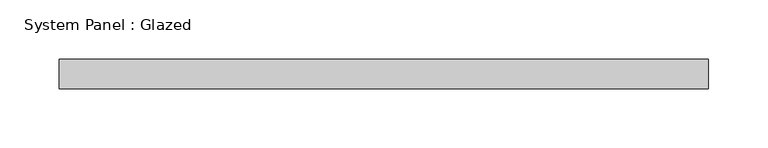
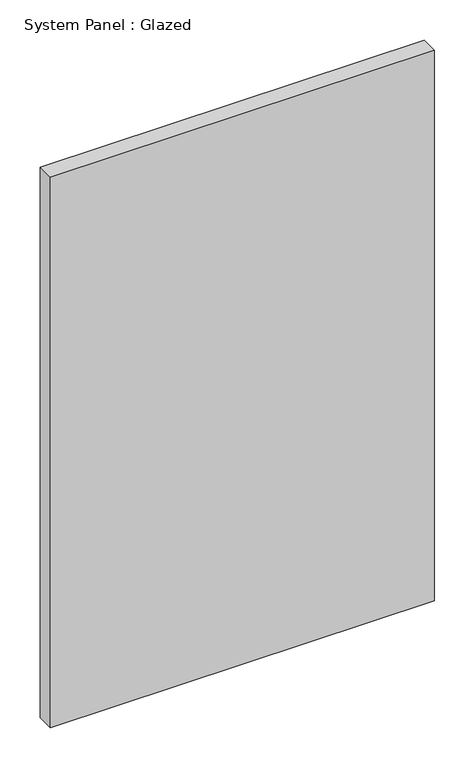
"""IFC4 building model written with IfcOpenShell, lengths in millimetres: plate geometry, System Panel : Glazed."""

from ifc_helpers import new_model, si_unit, origin, origin_with_axes, place, context, project, spatial, polyline, outline, extrude, source, transform, mapped, element, save


def system_panel_glazed_fb5ef4b2(model_context):
    return source(origin(), model_context, "Body", "SweptSolid", [
        extrude(outline(polyline([(275.0, 24.5), (-275.0, 24.5), (-275.0, 49.5), (275.0, 49.5), (275.0, 24.5)])), origin_with_axes(), (0.0, 0.0, 1.0), 833.3333333),
    ])


if __name__ == "__main__":
    model = new_model("IFC4")
    model_context = context("Model", 3, world=origin())
    ifc_project = project(units=[si_unit("LENGTHUNIT", "METRE", prefix="MILLI")], contexts=[model_context])
    site = spatial("IfcSite", under=ifc_project)
    building = spatial("IfcBuilding", under=site)
    placement = place(None, origin())
    system_panel_glazed_shape = system_panel_glazed_fb5ef4b2(model_context)
    element("IfcPlate", 1, ObjectType="System Panel : Glazed", at=placement, inside=building, context=model_context, shape_type="MappedRepresentation", body=[
        mapped(system_panel_glazed_shape, transform((0.0, 0.0, 0.0), x_axis=(1.0, 0.0, 0.0), y_axis=(0.0, 1.0, 0.0), z_axis=(0.0, 0.0, 1.0))),
    ])
    save(model, "model.ifc")

# Revit data of these elements
# Element 1 (IfcPlate, "System Panel : Glazed")
#   Materials on its faces: "Glass"
# Materials
#   "Glass": class "Glass", colour RGB 218 227 224, transparency 0.85, Description = "Soda Lime Glass", Cost = 0
